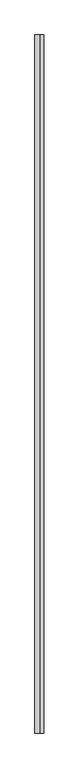
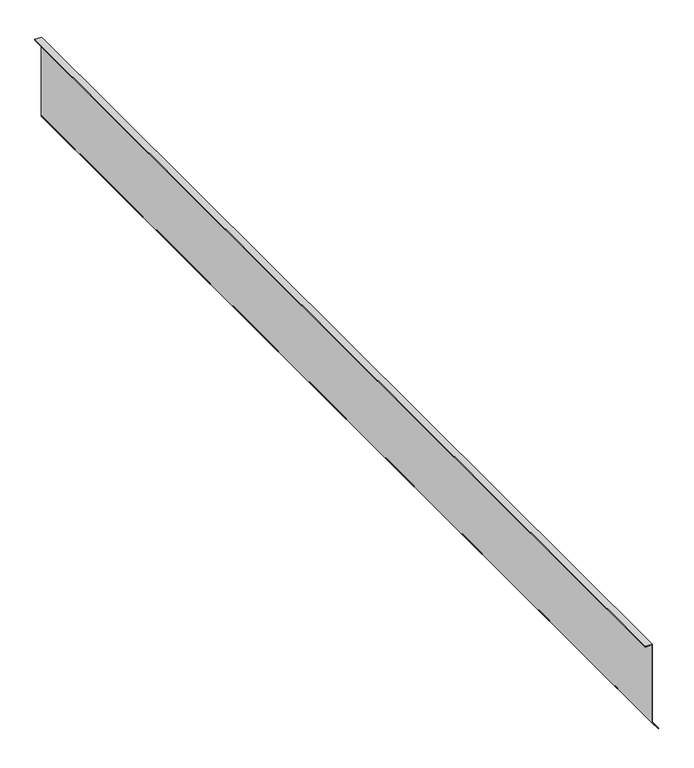
"""IFC4 building model written with IfcOpenShell, lengths in millimetres: proxy geometry, GRAVEL STOP004 3779 : GRAVEL STOP004 3779."""

from ifc_helpers import new_model, si_unit, frame, origin, place, context, project, spatial, polyline, outline, extrude, source, transform, mapped, element, save


def generic_models_78d96abb(model_context):
    return source(origin(), model_context, "Body", "SweptSolid", [
        extrude(outline(polyline([(40082.2407116, -4352.793241), (40097.9858473, -4365.3568119), (40254.7357103, -4365.3568119), (40254.7357103, -4378.5358417), (40253.3245993, -4378.5358417), (40253.3245993, -4366.7679229), (40097.4918556, -4366.7679229), (40081.3605882, -4353.8962446), (40082.2407116, -4352.793241)])), frame((0.0, -1065.5906573, 0.0), z_axis=(0.0, 1.0, 0.0), x_axis=(0.0, 0.0, 1.0)), (0.0, 0.0, 1.0), 2000.25),
    ])


if __name__ == "__main__":
    model = new_model("IFC4")
    model_context = context("Model", 3, world=origin())
    ifc_project = project(units=[si_unit("LENGTHUNIT", "METRE", prefix="MILLI")], contexts=[model_context])
    site = spatial("IfcSite", under=ifc_project)
    building = spatial("IfcBuilding", under=site)
    placement = place(None, origin())
    generic_models_shape = generic_models_78d96abb(model_context)
    element("IfcBuildingElementProxy", 1, Name="GRAVEL STOP004 3779 : GRAVEL STOP004 3779", ObjectType="GRAVEL STOP004 3779 : GRAVEL STOP004 3779", at=placement, inside=building, context=model_context, shape_type="MappedRepresentation", body=[
        mapped(generic_models_shape, transform((0.0, 0.0, 0.0), x_axis=(1.0, 0.0, 0.0), y_axis=(0.0, 1.0, 0.0), z_axis=(0.0, 0.0, 1.0))),
    ])
    save(model, "model.ifc")

# Revit data of these elements
# Type "GRAVEL STOP004 3779 : GRAVEL STOP004 3779"
#   NameOverride = "GRAVEL STOP004"
# Element 1 (IfcBuildingElementProxy, "GRAVEL STOP004 3779 : GRAVEL STOP004 3779")
#   Materials on its faces: "GRAVEL STOP REQUIRED WITH GRAVEL SURFACE SYSTEMS"
# Materials
#   "GRAVEL STOP REQUIRED WITH GRAVEL SURFACE SYSTEMS": class "Unassigned", colour RGB 170 170 127, transparency 0
